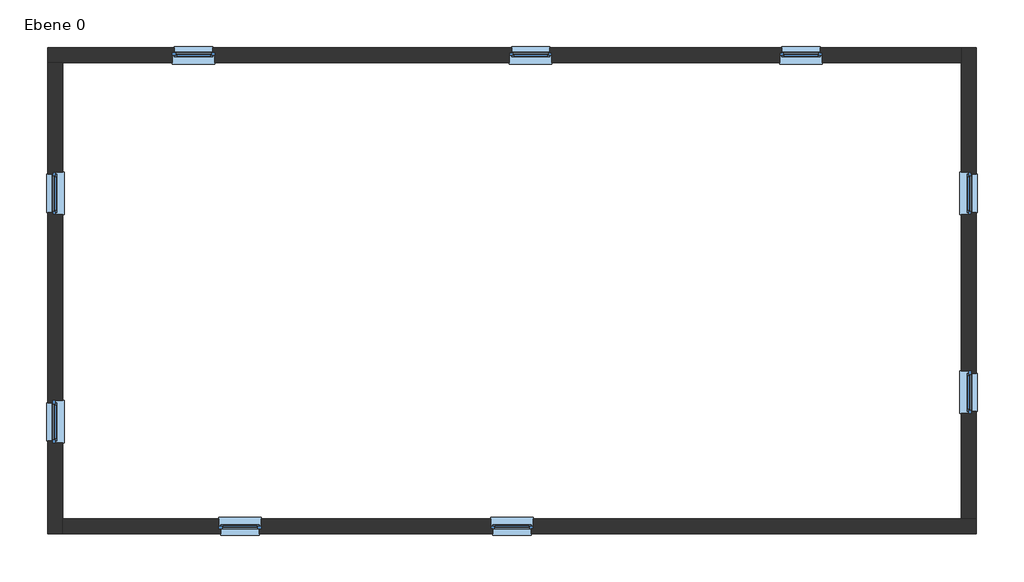
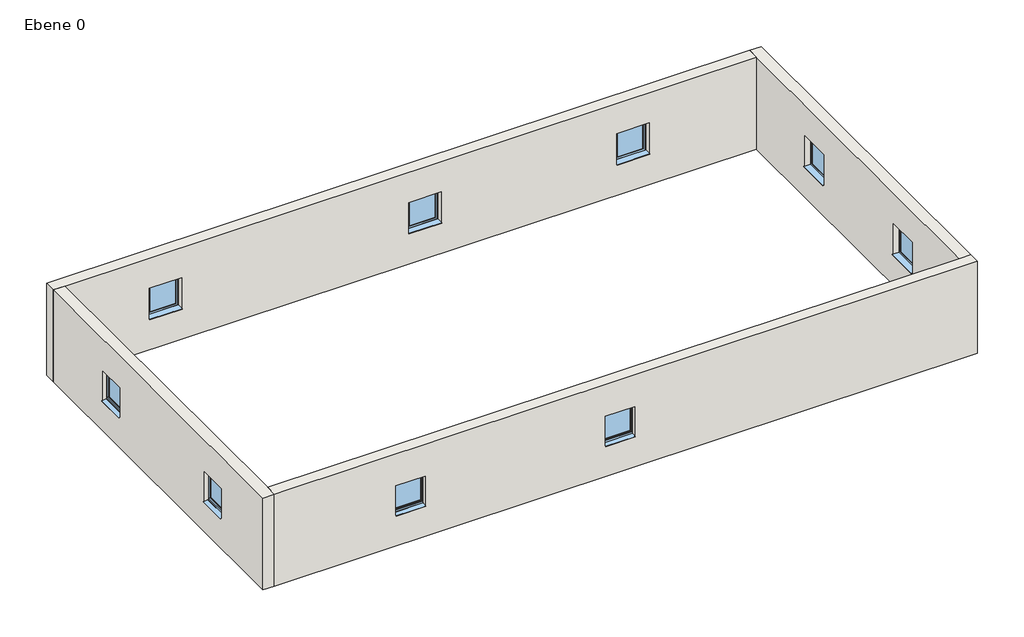
# One storey: 9 windows, 4 walls.
"""IFC4 building model written with IfcOpenShell, lengths in millimetres."""

import ifcopenshell
import ifcopenshell.guid

model = None  # the IFC model being written
_history = None  # IfcOwnerHistory: only IFC2X3 demands one
_inside = {}  # id of a spatial element -> (the spatial element, [elements in it])
_under = {}  # id of a project, library or spatial element -> (it, [spatial elements below it])
_declared = {}  # id of a project -> (the project, [libraries it declares])
_typed = {}  # id of a type object -> (the type object, [elements of that type])
_made_of = {}  # id of a material, layer set ... -> (it, [elements and type objects made of it])


def new_model(schema):
    """Start an empty IFC model of exactly this schema.

    Asked for "IFC4X3", IfcOpenShell would pick the latest addendum, in which some entities
    have other attributes; the version numbers below select the first issue.
    IFC2X3 requires an IfcOwnerHistory on every rooted entity: one is made here for all.
    """
    global model, _history
    if schema == "IFC4X3":
        model = ifcopenshell.file(schema_version=(4, 3, 0, 0))
    else:
        model = ifcopenshell.file(schema=schema)
    _inside.clear()
    _under.clear()
    _declared.clear()
    _typed.clear()
    _made_of.clear()
    _history = None
    if model.schema == "IFC2X3":
        org = make("IfcOrganization", Name="unknown")
        user = make(
            "IfcPersonAndOrganization",
            ThePerson=make("IfcPerson", FamilyName="unknown"),
            TheOrganization=org,
        )
        app = make(
            "IfcApplication",
            ApplicationDeveloper=org,
            Version="unknown",
            ApplicationFullName="unknown",
            ApplicationIdentifier="unknown",
        )
        _history = make(
            "IfcOwnerHistory",
            OwningUser=user,
            OwningApplication=app,
            ChangeAction="ADDED",
            CreationDate=0,
        )
    return model


def make(cls, **values):
    """One entity of the class cls with the attributes given. An attribute that is None is left unset."""
    return model.create_entity(
        cls, **{name: value for name, value in values.items() if value is not None}
    )


def rooted(cls, **values):
    """An entity with a GlobalId (a new one), such as an element, a storey or a relation."""
    return make(cls, GlobalId=ifcopenshell.guid.new(), OwnerHistory=_history, **values)


def si_unit(unit_type, name, prefix=None):
    """IfcSIUnit, for example si_unit("LENGTHUNIT", "METRE", prefix="MILLI")."""
    return make("IfcSIUnit", UnitType=unit_type, Prefix=prefix, Name=name)


def assignment(units):
    """IfcUnitAssignment: the units of a project."""
    return None if units is None else make("IfcUnitAssignment", Units=units)


def point(xyz):
    """IfcCartesianPoint."""
    return None if xyz is None else make("IfcCartesianPoint", Coordinates=xyz)


def direction(xyz):
    """IfcDirection."""
    return None if xyz is None else make("IfcDirection", DirectionRatios=xyz)


def frame(location, z_axis=None, x_axis=None):
    """IfcAxis2Placement3D, a coordinate frame: its origin and axes. An axis left out is left unset."""
    return make(
        "IfcAxis2Placement3D",
        Location=point(location),
        Axis=direction(z_axis),
        RefDirection=direction(x_axis),
    )


def origin():
    """The frame at (0, 0, 0) with its axes left unset."""
    return frame((0.0, 0.0, 0.0))


def place(relative_to, where):
    """IfcLocalPlacement: puts the frame where relative to a parent placement (None: the world)."""
    return make(
        "IfcLocalPlacement", PlacementRelTo=relative_to, RelativePlacement=where
    )


def context(
    kind, dimensions, precision=None, world=None, true_north=None, identifier=None
):
    """IfcGeometricRepresentationContext, for example the 3D "Model" context."""
    return make(
        "IfcGeometricRepresentationContext",
        ContextIdentifier=identifier,
        ContextType=kind,
        CoordinateSpaceDimension=dimensions,
        Precision=precision,
        WorldCoordinateSystem=world,
        TrueNorth=true_north,
    )


def project(units=None, contexts=None):
    """IfcProject with its units and contexts."""
    return rooted(
        "IfcProject",
        Name="project",
        RepresentationContexts=contexts,
        UnitsInContext=assignment(units),
    )


def spatial(cls, under=None, at=None, **own):
    """A site, building, storey or space (cls), placed at a placement, below another one or the project."""
    s = rooted(cls, ObjectPlacement=at, **own)
    if under is not None:
        _under.setdefault(under.id(), (under, []))[1].append(s)
    return s


def polyline(points):
    """IfcPolyline through the points."""
    return make("IfcPolyline", Points=[point(p) for p in points])


def outline(outer, holes=None, kind="AREA"):
    """IfcArbitraryClosedProfileDef: a profile drawn as a closed curve; with holes, ...WithVoids."""
    if holes is None:
        return make("IfcArbitraryClosedProfileDef", ProfileType=kind, OuterCurve=outer)
    return make(
        "IfcArbitraryProfileDefWithVoids",
        ProfileType=kind,
        OuterCurve=outer,
        InnerCurves=holes,
    )


def extrude(swept, where, along, depth):
    """IfcExtrudedAreaSolid: the profile swept, set in the frame where, extruded along a direction by depth."""
    return make(
        "IfcExtrudedAreaSolid",
        SweptArea=swept,
        Position=where,
        ExtrudedDirection=direction(along),
        Depth=depth,
    )


def faces_of(points, faces, orient=None, outer=None):
    """IfcFace entities. A face is a list of loops; a loop is a list of indices into points, from 0.

    orient and outer hold one flag for each loop. By default every Orientation is true, the
    first loop of a face is its IfcFaceOuterBound and the others are IfcFaceBound.
    """
    made = []
    for i, loops in enumerate(faces):
        bounds = []
        for j, loop in enumerate(loops):
            is_outer = j == 0 if outer is None else outer[i][j]
            bounds.append(
                make(
                    "IfcFaceOuterBound" if is_outer else "IfcFaceBound",
                    Bound=make("IfcPolyLoop", Polygon=[points[k] for k in loop]),
                    Orientation=True if orient is None else orient[i][j],
                )
            )
        made.append(make("IfcFace", Bounds=bounds))
    return made


def faceted_brep(points, faces, orient=None, outer=None, voids=None):
    """IfcFacetedBrep: a solid bounded by flat faces; with voids (closed shells), ...WithVoids."""
    shared = [point(p) for p in points]
    hull = make("IfcClosedShell", CfsFaces=faces_of(shared, faces, orient, outer))
    if voids is None:
        return make("IfcFacetedBrep", Outer=hull)
    return make(
        "IfcFacetedBrepWithVoids",
        Outer=hull,
        Voids=[
            make(cls, CfsFaces=faces_of(shared, fs, o, b)) for cls, fs, o, b in voids
        ],
    )


def shape(context_of_items, identifier, shape_type, items):
    """IfcShapeRepresentation: the items that make up one representation, for example the "Body"."""
    return make(
        "IfcShapeRepresentation",
        ContextOfItems=context_of_items,
        RepresentationIdentifier=identifier,
        RepresentationType=shape_type,
        Items=items,
    )


def source(mapping_origin, context_of_items, identifier, shape_type, items):
    """IfcRepresentationMap: a shape defined once, which mapped items show again and again."""
    return make(
        "IfcRepresentationMap",
        MappingOrigin=mapping_origin,
        MappedRepresentation=shape(context_of_items, identifier, shape_type, items),
    )


def transform(
    local_origin,
    x_axis=None,
    y_axis=None,
    z_axis=None,
    scale=None,
    scale2=None,
    scale3=None,
    uniform=True,
):
    """IfcCartesianTransformationOperator3D, or its non-uniform kind. x_axis, y_axis, z_axis: its Axis1, 2, 3."""
    if uniform:
        return make(
            "IfcCartesianTransformationOperator3D",
            Axis1=direction(x_axis),
            Axis2=direction(y_axis),
            LocalOrigin=point(local_origin),
            Scale=scale,
            Axis3=direction(z_axis),
        )
    return make(
        "IfcCartesianTransformationOperator3DnonUniform",
        Axis1=direction(x_axis),
        Axis2=direction(y_axis),
        LocalOrigin=point(local_origin),
        Scale=scale,
        Axis3=direction(z_axis),
        Scale2=scale2,
        Scale3=scale3,
    )


def mapped(mapping_source, mapping_target):
    """IfcMappedItem: shows the shape of a source again, moved by a transform."""
    return make(
        "IfcMappedItem", MappingSource=mapping_source, MappingTarget=mapping_target
    )


def made_of(thing, what):
    """Note that an element or type object is made of a material, layer set ...; save() writes the relation."""
    if what is not None:
        _made_of.setdefault(what.id(), (what, []))[1].append(thing)
    return thing


def element(
    cls,
    number,
    at=None,
    inside=None,
    cuts=None,
    type_object=None,
    material=None,
    context=None,
    identifier="Body",
    shape_type=None,
    held_by="IfcProductDefinitionShape",
    body=None,
    shapes=None,
    **own,
):
    """One element of the class cls, such as IfcWall. Its Tag is "e" and its number.

    at: its placement. inside: the storey or other place that contains it. cuts: it is an
    opening in that element (IfcRelVoidsElement). A single representation is given by context,
    identifier, shape_type and body (its items); several are given by shapes. held_by: the class
    of the entity that holds the representations. save() writes the other relations.
    """
    e = rooted(cls, Tag="e%d" % number, ObjectPlacement=at, **own)
    if body is not None:
        shapes = [shape(context, identifier, shape_type, body)]
    if shapes is not None:
        e.Representation = make(held_by, Representations=shapes)
    if inside is not None:
        _inside.setdefault(inside.id(), (inside, []))[1].append(e)
    if cuts is not None:
        rooted(
            "IfcRelVoidsElement", RelatingBuildingElement=cuts, RelatedOpeningElement=e
        )
    if type_object is not None:
        _typed.setdefault(type_object.id(), (type_object, []))[1].append(e)
    return made_of(e, material)


def aggregate(whole, parts):
    """IfcRelAggregates: a whole, such as a stair, and the parts it consists of."""
    return rooted("IfcRelAggregates", RelatingObject=whole, RelatedObjects=parts)


def save(model, path):
    """Write the relations noted so far, then the file.

    IfcRelAggregates (storeys below a building ...), IfcRelContainedInSpatialStructure (elements
    in a storey), IfcRelDefinesByType, IfcRelAssociatesMaterial and IfcRelDeclares: one each for
    every whole, place, type object, material and project.
    """
    for whole, parts in _under.values():
        aggregate(whole, parts)
    for where, things in _inside.values():
        rooted(
            "IfcRelContainedInSpatialStructure",
            RelatedElements=things,
            RelatingStructure=where,
        )
    for kind, things in _typed.values():
        rooted("IfcRelDefinesByType", RelatedObjects=things, RelatingType=kind)
    for what, things in _made_of.values():
        rooted("IfcRelAssociatesMaterial", RelatedObjects=things, RelatingMaterial=what)
    for by, libraries in _declared.values():
        rooted("IfcRelDeclares", RelatingContext=by, RelatedDefinitions=libraries)
    model.write(path)


def window_1_01_x_1_01_b7243dc8(model_context):
    return source(origin(), model_context, "Body", "SolidModel", [
        extrude(outline(polyline([(-525.0, -210.0), (-525.0, 0.0), (485.0, 0.0), (485.0, -210.0), (-525.0, -210.0)])), frame((0.0, 0.0, 1005.0), z_axis=(0.0, 0.0, 1.0), x_axis=(1.0, 0.0, 0.0)), (0.0, 0.0, 1.0), 15.0),
        extrude(outline(polyline([(375.0, -15.0), (-415.0, -15.0), (-415.0, 15.0), (375.0, 15.0), (375.0, -15.0)])), frame((0.0, 0.0, 1110.0), z_axis=(0.0, 0.0, 1.0), x_axis=(1.0, 0.0, 0.0)), (0.0, 0.0, 1.0), 790.0),
        extrude(outline(polyline([(70.0221543, 1020.0), (210.0, 1000.0), (210.0, 990.0), (208.0, 990.0), (208.0, 998.3604634), (69.8240723, 1018.0), (60.0, 1018.0), (60.0, 1020.0), (70.0221543, 1020.0)])), frame((-475.0, 0.0, 0.0), z_axis=(1.0, 0.0, 0.0), x_axis=(0.0, 1.0, 0.0)), (0.0, 0.0, 1.0), 910.0),
        extrude(outline(polyline([(2010.0, 485.0), (2010.0, -525.0), (1000.0, -525.0), (1000.0, 485.0), (2010.0, 485.0)]), holes=[polyline([(1930.0, 405.0), (1080.0, 405.0), (1080.0, -445.0), (1930.0, -445.0), (1930.0, 405.0)])]), frame((0.0, 0.0, 0.0), z_axis=(0.0, 1.0, 0.0), x_axis=(0.0, 0.0, 1.0)), (0.0, 0.0, 1.0), 60.0),
        faceted_brep([(435.0, 0.0, 1960.0), (435.0, -30.0, 1960.0), (435.0, -30.0, 1050.0), (435.0, 0.0, 1050.0), (-475.0, -30.0, 1960.0), (-475.0, -30.0, 1050.0), (375.0, -30.0, 1110.0), (-415.0, -30.0, 1110.0), (-415.0, -30.0, 1900.0), (375.0, -30.0, 1900.0), (-475.0, 0.0, 1050.0), (-475.0, 0.0, 1960.0), (405.0, 0.0, 1930.0), (-445.0, 0.0, 1930.0), (-445.0, 0.0, 1080.0), (405.0, 0.0, 1080.0), (405.0, 30.0, 1930.0), (405.0, 30.0, 1080.0), (-445.0, 30.0, 1080.0), (-445.0, 30.0, 1930.0), (375.0, 30.0, 1900.0), (-415.0, 30.0, 1900.0), (-415.0, 30.0, 1110.0), (375.0, 30.0, 1110.0)], [[[0, 1, 2, 3]], [[1, 4, 5, 2], [6, 7, 8, 9]], [[3, 2, 5, 10]], [[3, 10, 11, 0], [12, 13, 14, 15]], [[16, 12, 15, 17]], [[17, 15, 14, 18]], [[17, 18, 19, 16], [20, 21, 22, 23]], [[9, 20, 23, 6]], [[6, 23, 22, 7]], [[10, 5, 4, 11]], [[18, 14, 13, 19]], [[7, 22, 21, 8]], [[11, 4, 1, 0]], [[19, 13, 12, 16]], [[8, 21, 20, 9]]]),
    ])


model = new_model("IFC4")

# Units and contexts
model_context = context("Model", 3, world=origin())
ifc_project = project(units=[si_unit("LENGTHUNIT", "METRE", prefix="MILLI")], contexts=[model_context])

# Site, building, storey
site = spatial("IfcSite", under=ifc_project)
building = spatial("IfcBuilding", under=site)
storey = spatial("IfcBuildingStorey", under=building, Name="Ebene 0", Elevation=0.0)

# Walls
placement = place(None, origin())
element("IfcWall", 1, ObjectType="MW 24.0 WD 12.0", at=placement, inside=storey, context=model_context, shape_type="Brep", body=[
    faceted_brep([(-13369.6797169, 6985.6067473, 0.0), (-13009.6797169, 6985.6067473, 0.0), (8330.3202831, 6985.6067473, 0.0), (8330.3202831, 6985.6067473, 3000.0), (-13009.6797169, 6985.6067473, 3000.0), (-13369.6797169, 6985.6067473, 3000.0), (-9399.6797169, 6985.6067473, 1000.0), (-10409.6797169, 6985.6067473, 1000.0), (-10409.6797169, 6985.6067473, 2010.0), (-9399.6797169, 6985.6067473, 2010.0), (-1389.6797169, 6985.6067473, 1000.0), (-2399.6797169, 6985.6067473, 1000.0), (-2399.6797169, 6985.6067473, 2010.0), (-1389.6797169, 6985.6067473, 2010.0), (5030.3202831, 6985.6067473, 1000.0), (4020.3202831, 6985.6067473, 1000.0), (4020.3202831, 6985.6067473, 2010.0), (5030.3202831, 6985.6067473, 2010.0), (-13369.6797169, 7345.6067473, 0.0), (-13369.6797169, 7345.6067473, 3000.0), (8330.3202831, 7345.6067473, 3000.0), (8330.3202831, 7345.6067473, 0.0), (-9449.6797169, 7345.6067473, 1960.0), (-10359.6797169, 7345.6067473, 1960.0), (-10359.6797169, 7345.6067473, 1000.0), (-9449.6797169, 7345.6067473, 1000.0), (-1439.6797169, 7345.6067473, 1960.0), (-2349.6797169, 7345.6067473, 1960.0), (-2349.6797169, 7345.6067473, 1000.0), (-1439.6797169, 7345.6067473, 1000.0), (4980.3202831, 7345.6067473, 1960.0), (4070.3202831, 7345.6067473, 1960.0), (4070.3202831, 7345.6067473, 1000.0), (4980.3202831, 7345.6067473, 1000.0), (-9449.6797169, 7225.6067473, 1960.0), (-10359.6797169, 7225.6067473, 1960.0), (-10359.6797169, 7225.6067473, 1000.0), (-9449.6797169, 7225.6067473, 1000.0), (-10409.6797169, 7225.6067473, 1000.0), (-9399.6797169, 7225.6067473, 1000.0), (-10409.6797169, 7225.6067473, 2010.0), (-9399.6797169, 7225.6067473, 2010.0), (-1439.6797169, 7225.6067473, 1960.0), (-2349.6797169, 7225.6067473, 1960.0), (-2349.6797169, 7225.6067473, 1000.0), (-1439.6797169, 7225.6067473, 1000.0), (-2399.6797169, 7225.6067473, 1000.0), (-1389.6797169, 7225.6067473, 1000.0), (-2399.6797169, 7225.6067473, 2010.0), (-1389.6797169, 7225.6067473, 2010.0), (4980.3202831, 7225.6067473, 1960.0), (4070.3202831, 7225.6067473, 1960.0), (4070.3202831, 7225.6067473, 1000.0), (4980.3202831, 7225.6067473, 1000.0), (4020.3202831, 7225.6067473, 1000.0), (5030.3202831, 7225.6067473, 1000.0), (4020.3202831, 7225.6067473, 2010.0), (5030.3202831, 7225.6067473, 2010.0)], [[[0, 1, 2, 3, 4, 5], [6, 7, 8, 9], [10, 11, 12, 13], [14, 15, 16, 17]], [[18, 19, 20, 21], [22, 23, 24, 25], [26, 27, 28, 29], [30, 31, 32, 33]], [[2, 1, 0, 18, 21]], [[5, 4, 3, 20, 19]], [[0, 5, 19, 18]], [[3, 2, 21, 20]], [[22, 34, 35, 23]], [[23, 35, 36, 24]], [[34, 22, 25, 37]], [[24, 36, 38, 7, 6, 39, 37, 25]], [[40, 41, 9, 8]], [[41, 39, 6, 9]], [[41, 40, 38, 36, 35, 34, 37, 39]], [[38, 40, 8, 7]], [[26, 42, 43, 27]], [[27, 43, 44, 28]], [[42, 26, 29, 45]], [[28, 44, 46, 11, 10, 47, 45, 29]], [[48, 49, 13, 12]], [[49, 47, 10, 13]], [[49, 48, 46, 44, 43, 42, 45, 47]], [[46, 48, 12, 11]], [[30, 50, 51, 31]], [[31, 51, 52, 32]], [[50, 30, 33, 53]], [[32, 52, 54, 15, 14, 55, 53, 33]], [[56, 57, 17, 16]], [[57, 55, 14, 17]], [[57, 56, 54, 52, 51, 50, 53, 55]], [[54, 56, 16, 15]]]),
])
element("IfcWall", 2, ObjectType="MW 24.0 WD 12.0", at=placement, inside=storey, context=model_context, shape_type="Brep", body=[
    faceted_brep([(-13009.6797169, -4214.3932527, 0.0), (-13009.6797169, -3854.3932527, 0.0), (-13009.6797169, 6985.6067473, 0.0), (-13009.6797169, 6985.6067473, 3000.0), (-13009.6797169, -3854.3932527, 3000.0), (-13009.6797169, -4214.3932527, 3000.0), (-13009.6797169, -1044.3932527, 1000.0), (-13009.6797169, -2054.3932527, 1000.0), (-13009.6797169, -2054.3932527, 2010.0), (-13009.6797169, -1044.3932527, 2010.0), (-13009.6797169, 4385.6067473, 1000.0), (-13009.6797169, 3375.6067473, 1000.0), (-13009.6797169, 3375.6067473, 2010.0), (-13009.6797169, 4385.6067473, 2010.0), (-13369.6797169, -4214.3932527, 0.0), (-13369.6797169, -4214.3932527, 3000.0), (-13369.6797169, 6985.6067473, 3000.0), (-13369.6797169, 6985.6067473, 0.0), (-13369.6797169, -1094.3932527, 1960.0), (-13369.6797169, -2004.3932527, 1960.0), (-13369.6797169, -2004.3932527, 1000.0), (-13369.6797169, -1094.3932527, 1000.0), (-13369.6797169, 4335.6067473, 1960.0), (-13369.6797169, 3425.6067473, 1960.0), (-13369.6797169, 3425.6067473, 1000.0), (-13369.6797169, 4335.6067473, 1000.0), (-13249.6797169, -1094.3932527, 1960.0), (-13249.6797169, -2004.3932527, 1960.0), (-13249.6797169, -2004.3932527, 1000.0), (-13249.6797169, -1094.3932527, 1000.0), (-13249.6797169, -2054.3932527, 1000.0), (-13249.6797169, -1044.3932527, 1000.0), (-13249.6797169, -2054.3932527, 2010.0), (-13249.6797169, -1044.3932527, 2010.0), (-13249.6797169, 4335.6067473, 1960.0), (-13249.6797169, 3425.6067473, 1960.0), (-13249.6797169, 3425.6067473, 1000.0), (-13249.6797169, 4335.6067473, 1000.0), (-13249.6797169, 3375.6067473, 1000.0), (-13249.6797169, 4385.6067473, 1000.0), (-13249.6797169, 3375.6067473, 2010.0), (-13249.6797169, 4385.6067473, 2010.0)], [[[0, 1, 2, 3, 4, 5], [6, 7, 8, 9], [10, 11, 12, 13]], [[14, 15, 16, 17], [18, 19, 20, 21], [22, 23, 24, 25]], [[2, 1, 0, 14, 17]], [[5, 4, 3, 16, 15]], [[0, 5, 15, 14]], [[3, 2, 17, 16]], [[18, 26, 27, 19]], [[19, 27, 28, 20]], [[26, 18, 21, 29]], [[20, 28, 30, 7, 6, 31, 29, 21]], [[32, 33, 9, 8]], [[33, 31, 6, 9]], [[33, 32, 30, 28, 27, 26, 29, 31]], [[30, 32, 8, 7]], [[22, 34, 35, 23]], [[23, 35, 36, 24]], [[34, 22, 25, 37]], [[24, 36, 38, 11, 10, 39, 37, 25]], [[40, 41, 13, 12]], [[41, 39, 10, 13]], [[41, 40, 38, 36, 35, 34, 37, 39]], [[38, 40, 12, 11]]]),
])
element("IfcWall", 3, ObjectType="MW 24.0 WD 12.0", at=placement, inside=storey, context=model_context, shape_type="Brep", body=[
    faceted_brep([(8690.3202831, -3854.3932527, 0.0), (8330.3202831, -3854.3932527, 0.0), (-13009.6797169, -3854.3932527, 0.0), (-13009.6797169, -3854.3932527, 3000.0), (8330.3202831, -3854.3932527, 3000.0), (8690.3202831, -3854.3932527, 3000.0), (-2844.6797169, -3854.3932527, 1000.0), (-1834.6797169, -3854.3932527, 1000.0), (-1834.6797169, -3854.3932527, 2010.0), (-2844.6797169, -3854.3932527, 2010.0), (-9309.6797169, -3854.3932527, 1000.0), (-8299.6797169, -3854.3932527, 1000.0), (-8299.6797169, -3854.3932527, 2010.0), (-9309.6797169, -3854.3932527, 2010.0), (8690.3202831, -4214.3932527, 0.0), (8690.3202831, -4214.3932527, 3000.0), (-13009.6797169, -4214.3932527, 3000.0), (-13009.6797169, -4214.3932527, 0.0), (-2794.6797169, -4214.3932527, 1960.0), (-1884.6797169, -4214.3932527, 1960.0), (-1884.6797169, -4214.3932527, 1000.0), (-2794.6797169, -4214.3932527, 1000.0), (-9259.6797169, -4214.3932527, 1960.0), (-8349.6797169, -4214.3932527, 1960.0), (-8349.6797169, -4214.3932527, 1000.0), (-9259.6797169, -4214.3932527, 1000.0), (-2794.6797169, -4094.3932527, 1960.0), (-1884.6797169, -4094.3932527, 1960.0), (-1884.6797169, -4094.3932527, 1000.0), (-2794.6797169, -4094.3932527, 1000.0), (-1834.6797169, -4094.3932527, 1000.0), (-2844.6797169, -4094.3932527, 1000.0), (-1834.6797169, -4094.3932527, 2010.0), (-2844.6797169, -4094.3932527, 2010.0), (-9259.6797169, -4094.3932527, 1960.0), (-8349.6797169, -4094.3932527, 1960.0), (-8349.6797169, -4094.3932527, 1000.0), (-9259.6797169, -4094.3932527, 1000.0), (-8299.6797169, -4094.3932527, 1000.0), (-9309.6797169, -4094.3932527, 1000.0), (-8299.6797169, -4094.3932527, 2010.0), (-9309.6797169, -4094.3932527, 2010.0)], [[[0, 1, 2, 3, 4, 5], [6, 7, 8, 9], [10, 11, 12, 13]], [[14, 15, 16, 17], [18, 19, 20, 21], [22, 23, 24, 25]], [[2, 1, 0, 14, 17]], [[5, 4, 3, 16, 15]], [[0, 5, 15, 14]], [[3, 2, 17, 16]], [[18, 26, 27, 19]], [[19, 27, 28, 20]], [[26, 18, 21, 29]], [[20, 28, 30, 7, 6, 31, 29, 21]], [[32, 33, 9, 8]], [[33, 31, 6, 9]], [[33, 32, 30, 28, 27, 26, 29, 31]], [[30, 32, 8, 7]], [[22, 34, 35, 23]], [[23, 35, 36, 24]], [[34, 22, 25, 37]], [[24, 36, 38, 11, 10, 39, 37, 25]], [[40, 41, 13, 12]], [[41, 39, 10, 13]], [[41, 40, 38, 36, 35, 34, 37, 39]], [[38, 40, 12, 11]]]),
])
element("IfcWall", 4, ObjectType="MW 24.0 WD 12.0", at=placement, inside=storey, context=model_context, shape_type="Brep", body=[
    faceted_brep([(8330.3202831, 7345.6067473, 0.0), (8330.3202831, 6985.6067473, 0.0), (8330.3202831, -3854.3932527, 0.0), (8330.3202831, -3854.3932527, 3000.0), (8330.3202831, 6985.6067473, 3000.0), (8330.3202831, 7345.6067473, 3000.0), (8330.3202831, 3375.6067473, 1000.0), (8330.3202831, 4385.6067473, 1000.0), (8330.3202831, 4385.6067473, 2010.0), (8330.3202831, 3375.6067473, 2010.0), (8330.3202831, -1354.3932527, 1000.0), (8330.3202831, -344.3932527, 1000.0), (8330.3202831, -344.3932527, 2010.0), (8330.3202831, -1354.3932527, 2010.0), (8690.3202831, 7345.6067473, 0.0), (8690.3202831, 7345.6067473, 3000.0), (8690.3202831, -3854.3932527, 3000.0), (8690.3202831, -3854.3932527, 0.0), (8690.3202831, 3425.6067473, 1960.0), (8690.3202831, 4335.6067473, 1960.0), (8690.3202831, 4335.6067473, 1000.0), (8690.3202831, 3425.6067473, 1000.0), (8690.3202831, -1304.3932527, 1960.0), (8690.3202831, -394.3932527, 1960.0), (8690.3202831, -394.3932527, 1000.0), (8690.3202831, -1304.3932527, 1000.0), (8570.3202831, 3425.6067473, 1960.0), (8570.3202831, 4335.6067473, 1960.0), (8570.3202831, 4335.6067473, 1000.0), (8570.3202831, 3425.6067473, 1000.0), (8570.3202831, 4385.6067473, 1000.0), (8570.3202831, 3375.6067473, 1000.0), (8570.3202831, 4385.6067473, 2010.0), (8570.3202831, 3375.6067473, 2010.0), (8570.3202831, -1304.3932527, 1960.0), (8570.3202831, -394.3932527, 1960.0), (8570.3202831, -394.3932527, 1000.0), (8570.3202831, -1304.3932527, 1000.0), (8570.3202831, -344.3932527, 1000.0), (8570.3202831, -1354.3932527, 1000.0), (8570.3202831, -344.3932527, 2010.0), (8570.3202831, -1354.3932527, 2010.0)], [[[0, 1, 2, 3, 4, 5], [6, 7, 8, 9], [10, 11, 12, 13]], [[14, 15, 16, 17], [18, 19, 20, 21], [22, 23, 24, 25]], [[2, 1, 0, 14, 17]], [[5, 4, 3, 16, 15]], [[0, 5, 15, 14]], [[3, 2, 17, 16]], [[18, 26, 27, 19]], [[19, 27, 28, 20]], [[26, 18, 21, 29]], [[20, 28, 30, 7, 6, 31, 29, 21]], [[32, 33, 9, 8]], [[33, 31, 6, 9]], [[33, 32, 30, 28, 27, 26, 29, 31]], [[30, 32, 8, 7]], [[22, 34, 35, 23]], [[23, 35, 36, 24]], [[34, 22, 25, 37]], [[24, 36, 38, 11, 10, 39, 37, 25]], [[40, 41, 13, 12]], [[41, 39, 10, 13]], [[41, 40, 38, 36, 35, 34, 37, 39]], [[38, 40, 12, 11]]]),
])

# Windows
window_1_01_x_1_01_shape = window_1_01_x_1_01_b7243dc8(model_context)
element("IfcWindow", 5, ObjectType="Fenster 1-flg - Anschlag : 1.01 x 1.01", at=placement, inside=storey, context=model_context, shape_type="MappedRepresentation", body=[
    mapped(window_1_01_x_1_01_shape, transform((-9884.6797169, 7165.6067473, 0.0), x_axis=(1.0, 0.0, 0.0), y_axis=(0.0, 1.0, 0.0), z_axis=(0.0, 0.0, 1.0))),
])
element("IfcWindow", 6, ObjectType="Fenster 1-flg - Anschlag : 1.01 x 1.01", at=placement, inside=storey, context=model_context, shape_type="MappedRepresentation", body=[
    mapped(window_1_01_x_1_01_shape, transform((-1874.6797169, 7165.6067473, 0.0), x_axis=(1.0, 0.0, 0.0), y_axis=(0.0, 1.0, 0.0), z_axis=(0.0, 0.0, 1.0))),
])
element("IfcWindow", 7, ObjectType="Fenster 1-flg - Anschlag : 1.01 x 1.01", at=placement, inside=storey, context=model_context, shape_type="MappedRepresentation", body=[
    mapped(window_1_01_x_1_01_shape, transform((4545.3202831, 7165.6067473, 0.0), x_axis=(1.0, 0.0, 0.0), y_axis=(0.0, 1.0, 0.0), z_axis=(0.0, 0.0, 1.0))),
])
element("IfcWindow", 8, ObjectType="Fenster 1-flg - Anschlag : 1.01 x 1.01", at=placement, inside=storey, context=model_context, shape_type="MappedRepresentation", body=[
    mapped(window_1_01_x_1_01_shape, transform((8510.3202831, 3860.6067473, 0.0), x_axis=(0.0, -1.0, 0.0), y_axis=(1.0, 0.0, 0.0), z_axis=(0.0, 0.0, 1.0))),
])
element("IfcWindow", 9, ObjectType="Fenster 1-flg - Anschlag : 1.01 x 1.01", at=placement, inside=storey, context=model_context, shape_type="MappedRepresentation", body=[
    mapped(window_1_01_x_1_01_shape, transform((8510.3202831, -869.3932527, 0.0), x_axis=(0.0, -1.0, 0.0), y_axis=(1.0, 0.0, 0.0), z_axis=(0.0, 0.0, 1.0))),
])
element("IfcWindow", 10, ObjectType="Fenster 1-flg - Anschlag : 1.01 x 1.01", at=placement, inside=storey, context=model_context, shape_type="MappedRepresentation", body=[
    mapped(window_1_01_x_1_01_shape, transform((-2359.6797169, -4034.3932527, 0.0), x_axis=(-1.0, 0.0, 0.0), y_axis=(0.0, -1.0, 0.0), z_axis=(0.0, 0.0, 1.0))),
])
element("IfcWindow", 11, ObjectType="Fenster 1-flg - Anschlag : 1.01 x 1.01", at=placement, inside=storey, context=model_context, shape_type="MappedRepresentation", body=[
    mapped(window_1_01_x_1_01_shape, transform((-8824.6797169, -4034.3932527, 0.0), x_axis=(-1.0, 0.0, 0.0), y_axis=(0.0, -1.0, 0.0), z_axis=(0.0, 0.0, 1.0))),
])
element("IfcWindow", 12, ObjectType="Fenster 1-flg - Anschlag : 1.01 x 1.01", at=placement, inside=storey, context=model_context, shape_type="MappedRepresentation", body=[
    mapped(window_1_01_x_1_01_shape, transform((-13189.6797169, -1529.3932527, 0.0), x_axis=(0.0, 1.0, 0.0), y_axis=(-1.0, 0.0, 0.0), z_axis=(0.0, 0.0, 1.0))),
])
element("IfcWindow", 13, ObjectType="Fenster 1-flg - Anschlag : 1.01 x 1.01", at=placement, inside=storey, context=model_context, shape_type="MappedRepresentation", body=[
    mapped(window_1_01_x_1_01_shape, transform((-13189.6797169, 3900.6067473, 0.0), x_axis=(0.0, 1.0, 0.0), y_axis=(-1.0, 0.0, 0.0), z_axis=(0.0, 0.0, 1.0))),
])

save(model, "model.ifc")

# Revit data of these elements
# Project information
#   Projektausgabedatum = "Projekt Datum"
#   Projektstatus = "Projektstatus"
#   Kundenname = "Bauherr"
#   Projektadresse = "Projektadresse"
#   Projektname = "Projektname"
#   Projektnummer = "Projektnummer"
#   Verfasser Firma 1 = "Firma 1"
#   Verfasser Firma 2 = "Firma 2"
#   Verfasser PLZ Ort = "PLZ Ort"
#   Verfasser Strasse = "Strasse"
#   Verfasser Telefon = "Telefon"
#   Verfasser Telefax = "Telefax"
#   Verfasser eMail = "E-Mail"
# Type "MW 24.0 WD 12.0"
#   Type Comments = "Mehrschaliges Mauerwerk"
#   Description = "Mauerwerk 24.0 cm, Wärmedämmung 12.0 cm"
#   Width = 0.360 m
#   Layers, outside or top first: 0.120 m "Wärmedämmung - Hart" (function 3); 0.240 m "Mauerwerk - Ziegel, verputzt" (function 1)
# Type "Fenster 1-flg - Anschlag : 1.01 x 1.01"
#   Type Mark = "47"
#   Operation = "SinglePanel"
#   Keynote = "16.05.01"
#   Construction Type Id = "GSP4R"
#   Analytic Construction = "1/8 Zoll Pilkington-Verglasung einfach"
#   Visual Light Transmittance = 0.9
#   Thermal Resistance (R) = 0.1491 (m²·K)/W
#   Solar Heat Gain Coefficient = 0.86
#   Anschlagsbreite seitlich = 0.050 m
#   Rough Width = 1.010 m
#   Rough Height = 1.010 m
#   Heat Transfer Coefficient (U) = 6.7069 W/(m²·K)
#   Rahmentiefe = 0.060 m
#   Rahmenhöhe unten = 0.080 m
#   Rahmenhöhe oben = 0.080 m
#   Rahmenbreite = 0.080 m
#   Height = 1.010 m
#   Flügeltiefe = 0.060 m
#   Flügelbreite = 0.060 m
#   Einbautiefe (von außen) [instance default] = 0.120 m
#   Width = 1.010 m
#   Anschlagsbreite oben = 0.050 m
#   Klappflügel [instance default] = no
#   Öffnungsrichtung oben [instance default] = yes
#   Öffnungsrichtung in Draufsicht anzeigen [instance default] = no
#   Drehflügel [instance default] = yes
#   Rahmen [instance default] = none
#   Glas [instance default] = none
#   Flügel [instance default] = none
#   Fensterbank innen [instance default] = none
#   Fensterbank außen [instance default] = none
#   Wall Closure = (empty or 0)
# Elements 1, 2, 3, 4 (IfcWall, "MW 24.0 WD 12.0")
#   Top Offset = 0.000 m
#   Base Offset = 0.000 m
#   wall height = 3.000 m
#   Phase Created = Phase 1
#   Base Constraint = Ebene 0
#   Top Constraint = Ebene 1
#   Materials on its faces: "Standard - Wand", "Wärmedämmung - Hart", "Mauerwerk - Ziegel, verputzt"
# Element 5 (IfcWindow, "Fenster 1-flg - Anschlag : 1.01 x 1.01")
#   Mark = "1"
#   Einbautiefe (von außen) = 0.120 m
#   Öffnungsrichtung oben = yes
#   Öffnungsrichtung in Draufsicht anzeigen = no
#   Klappflügel = no
#   Drehflügel = yes
#   Rahmen = none
#   Glas = none
#   Flügel = none
#   Fensterbank innen = none
#   Fensterbank außen = none
#   Phase Created = Phase 1
#   Materials on its faces: "Kunststoff - Weiß", "Holz - Birke", "Glas"
# Element 6 (IfcWindow, "Fenster 1-flg - Anschlag : 1.01 x 1.01")
#   Mark = "2"
#   Einbautiefe (von außen) = 0.120 m
#   Öffnungsrichtung oben = yes
#   Öffnungsrichtung in Draufsicht anzeigen = no
#   Klappflügel = no
#   Drehflügel = yes
#   Rahmen = none
#   Glas = none
#   Flügel = none
#   Fensterbank innen = none
#   Fensterbank außen = none
#   Phase Created = Phase 1
#   Materials on its faces: "Kunststoff - Weiß", "Holz - Birke", "Glas"
# Element 7 (IfcWindow, "Fenster 1-flg - Anschlag : 1.01 x 1.01")
#   Mark = "3"
#   Einbautiefe (von außen) = 0.120 m
#   Öffnungsrichtung oben = yes
#   Öffnungsrichtung in Draufsicht anzeigen = no
#   Klappflügel = no
#   Drehflügel = yes
#   Rahmen = none
#   Glas = none
#   Flügel = none
#   Fensterbank innen = none
#   Fensterbank außen = none
#   Phase Created = Phase 1
#   Materials on its faces: "Kunststoff - Weiß", "Holz - Birke", "Glas"
# Element 8 (IfcWindow, "Fenster 1-flg - Anschlag : 1.01 x 1.01")
#   Mark = "4"
#   Einbautiefe (von außen) = 0.120 m
#   Öffnungsrichtung oben = yes
#   Öffnungsrichtung in Draufsicht anzeigen = no
#   Klappflügel = no
#   Drehflügel = yes
#   Rahmen = none
#   Glas = none
#   Flügel = none
#   Fensterbank innen = none
#   Fensterbank außen = none
#   Phase Created = Phase 1
#   Materials on its faces: "Kunststoff - Weiß", "Holz - Birke", "Glas"
# Element 9 (IfcWindow, "Fenster 1-flg - Anschlag : 1.01 x 1.01")
#   Mark = "5"
#   Einbautiefe (von außen) = 0.120 m
#   Öffnungsrichtung oben = yes
#   Öffnungsrichtung in Draufsicht anzeigen = no
#   Klappflügel = no
#   Drehflügel = yes
#   Rahmen = none
#   Glas = none
#   Flügel = none
#   Fensterbank innen = none
#   Fensterbank außen = none
#   Phase Created = Phase 1
#   Materials on its faces: "Kunststoff - Weiß", "Holz - Birke", "Glas"
# Element 10 (IfcWindow, "Fenster 1-flg - Anschlag : 1.01 x 1.01")
#   Mark = "6"
#   Einbautiefe (von außen) = 0.120 m
#   Öffnungsrichtung oben = yes
#   Öffnungsrichtung in Draufsicht anzeigen = no
#   Klappflügel = no
#   Drehflügel = yes
#   Rahmen = none
#   Glas = none
#   Flügel = none
#   Fensterbank innen = none
#   Fensterbank außen = none
#   Phase Created = Phase 1
#   Materials on its faces: "Kunststoff - Weiß", "Holz - Birke", "Glas"
# Element 11 (IfcWindow, "Fenster 1-flg - Anschlag : 1.01 x 1.01")
#   Mark = "7"
#   Einbautiefe (von außen) = 0.120 m
#   Öffnungsrichtung oben = yes
#   Öffnungsrichtung in Draufsicht anzeigen = no
#   Klappflügel = no
#   Drehflügel = yes
#   Rahmen = none
#   Glas = none
#   Flügel = none
#   Fensterbank innen = none
#   Fensterbank außen = none
#   Phase Created = Phase 1
#   Materials on its faces: "Kunststoff - Weiß", "Holz - Birke", "Glas"
# Element 12 (IfcWindow, "Fenster 1-flg - Anschlag : 1.01 x 1.01")
#   Mark = "8"
#   Einbautiefe (von außen) = 0.120 m
#   Öffnungsrichtung oben = yes
#   Öffnungsrichtung in Draufsicht anzeigen = no
#   Klappflügel = no
#   Drehflügel = yes
#   Rahmen = none
#   Glas = none
#   Flügel = none
#   Fensterbank innen = none
#   Fensterbank außen = none
#   Phase Created = Phase 1
#   Materials on its faces: "Kunststoff - Weiß", "Holz - Birke", "Glas"
# Element 13 (IfcWindow, "Fenster 1-flg - Anschlag : 1.01 x 1.01")
#   Mark = "9"
#   Einbautiefe (von außen) = 0.120 m
#   Öffnungsrichtung oben = yes
#   Öffnungsrichtung in Draufsicht anzeigen = no
#   Klappflügel = no
#   Drehflügel = yes
#   Rahmen = none
#   Glas = none
#   Flügel = none
#   Fensterbank innen = none
#   Fensterbank außen = none
#   Phase Created = Phase 1
#   Materials on its faces: "Kunststoff - Weiß", "Holz - Birke", "Glas"
# Materials
#   "Wärmedämmung - Hart": class "Putz", colour RGB 255 255 255, transparency 0, Description = "Äußere Oberfläche"
#   "Mauerwerk - Ziegel, verputzt": class "Putz", colour RGB 247 247 247, transparency 0, Cost = 0
#   "Standard - Wand": class "Putz", colour RGB 128 128 128, transparency 0, Description = "Äußere Oberfläche"
#   "Kunststoff - Weiß": class "Kunststoff", colour RGB 249 249 249, transparency 0
#   "Holz - Birke": class "Holz", colour RGB 213 164 103, transparency 0
#   "Glas": class "Glas", colour RGB 0 0 255, transparency 0.75, Comments = "Renderdarstellung nicht aktualisiert ", Cost = 0
